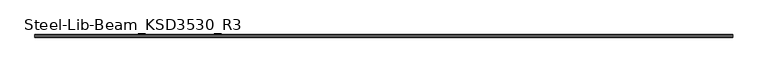
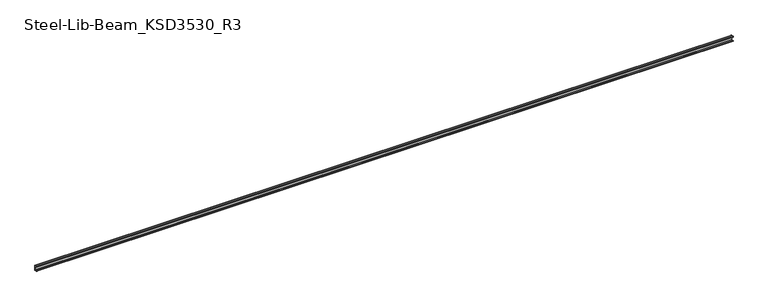
"""IFC4 building model written with IfcOpenShell, lengths in millimetres: beam geometry, Steel-Lib-Beam_KSD3530_R3 : BMS291_C-150×75x20x4.5."""

from ifc_helpers import new_model, si_unit, point, frame, frame_2d, origin, place, context, project, spatial, polyline, circle_curve, trimmed, segment, composite_curve, outline, extrude, source, transform, mapped, element, save


def steel_lib_beam_ksd3530_r3_05b44c44(model_context):
    return source(origin(), model_context, "Body", "SweptSolid", [
        extrude(outline(composite_curve([segment(trimmed(circle_curve(frame_2d((-41.0, 66.0)), 9.0), [point((-50.0, 66.0))], [point((-41.0, 75.0))], False, "CARTESIAN"), True, "CONTINUOUS"), segment(polyline([(-41.0, 75.0), (16.0, 75.0)]), True, "CONTINUOUS"), segment(trimmed(circle_curve(frame_2d((16.0, 66.0)), 9.0), [point((16.0, 75.0))], [point((25.0, 66.0))], False, "CARTESIAN"), True, "CONTINUOUS"), segment(polyline([(25.0, 66.0), (25.0, -66.0)]), True, "CONTINUOUS"), segment(trimmed(circle_curve(frame_2d((16.0, -66.0)), 9.0), [point((25.0, -66.0))], [point((16.0, -75.0))], False, "CARTESIAN"), True, "CONTINUOUS"), segment(polyline([(16.0, -75.0), (-41.0, -75.0)]), True, "CONTINUOUS"), segment(trimmed(circle_curve(frame_2d((-41.0, -66.0)), 9.0), [point((-41.0, -75.0))], [point((-50.0, -66.0))], False, "CARTESIAN"), True, "CONTINUOUS"), segment(polyline([(-50.0, -66.0), (-50.0, -55.0), (-45.5, -55.0), (-45.5, -66.0)]), True, "CONTINUOUS"), segment(trimmed(circle_curve(frame_2d((-41.0, -66.0)), 4.5), [point((-45.5, -66.0))], [point((-41.0, -70.5))], True, "CARTESIAN"), True, "CONTINUOUS"), segment(polyline([(-41.0, -70.5), (16.0, -70.5)]), True, "CONTINUOUS"), segment(trimmed(circle_curve(frame_2d((16.0, -66.0)), 4.5), [point((16.0, -70.5))], [point((20.5, -66.0))], True, "CARTESIAN"), True, "CONTINUOUS"), segment(polyline([(20.5, -66.0), (20.5, 66.0)]), True, "CONTINUOUS"), segment(trimmed(circle_curve(frame_2d((16.0, 66.0)), 4.5), [point((20.5, 66.0))], [point((16.0, 70.5))], True, "CARTESIAN"), True, "CONTINUOUS"), segment(polyline([(16.0, 70.5), (-41.0, 70.5)]), True, "CONTINUOUS"), segment(trimmed(circle_curve(frame_2d((-41.0, 66.0)), 4.5), [point((-41.0, 70.5))], [point((-45.5, 66.0))], True, "CARTESIAN"), True, "CONTINUOUS"), segment(polyline([(-45.5, 66.0), (-45.5, 55.0), (-50.0, 55.0), (-50.0, 66.0)]), True, "CONTINUOUS")], self_intersect=False)), frame((-9880.0, 0.0, 0.0), z_axis=(1.0, 0.0, 0.0), x_axis=(0.0, 1.0, 0.0)), (0.0, 0.0, 1.0), 19760.0),
    ])


if __name__ == "__main__":
    model = new_model("IFC4")
    model_context = context("Model", 3, world=origin())
    ifc_project = project(units=[si_unit("LENGTHUNIT", "METRE", prefix="MILLI")], contexts=[model_context])
    site = spatial("IfcSite", under=ifc_project)
    building = spatial("IfcBuilding", under=site)
    placement = place(None, origin())
    steel_lib_beam_ksd3530_r3_shape = steel_lib_beam_ksd3530_r3_05b44c44(model_context)
    element("IfcBeam", 1, ObjectType="Steel-Lib-Beam_KSD3530_R3 : BMS291_C-150×75x20x4.5", at=placement, inside=building, context=model_context, shape_type="MappedRepresentation", body=[
        mapped(steel_lib_beam_ksd3530_r3_shape, transform((0.0, 0.0, 0.0), x_axis=(1.0, 0.0, 0.0), y_axis=(0.0, 1.0, 0.0), z_axis=(0.0, 0.0, 1.0))),
    ])
    save(model, "model.ifc")

# Revit data of these elements
# Type "Steel-Lib-Beam_KSD3530_R3 : BMS291_C-150×75x20x4.5"
#   Keynote = "C-150×75x20x4.5"
#   SteelWeight = "Light"
#   x = 0.0250 m
#   t1 = 0.0090 m
#   t = 0.0045 m
#   Surface Area = 0.629834 m²/m
#   Section Area = 13.9688 cm²
#   Mass per Unit Length = 10.9655 kg/m
#   C = 0.0200 m
#   A = 0.0750 m
#   Length [instance default] = 1.5000 m
#   H = 0.1500 m
#   hec_material4 [instance default] = none
#   hec_material3 [instance default] = none
#   hec_material2 [instance default] = none
#   hec_material1 [instance default] = none
#   Structural Material [instance default] = Metal - Steel - Light Gauge
#   Assembly Code = ""
# Element 1 (IfcBeam, "Steel-Lib-Beam_KSD3530_R3 : BMS291_C-150×75x20x4.5")
#   Structural Material = none
# Materials
#   "Metal - Steel - Light Gauge": class "Metal", colour RGB 247 247 247, transparency 0
